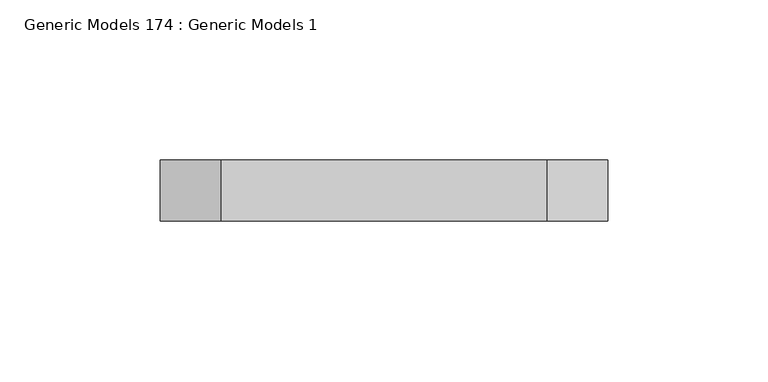
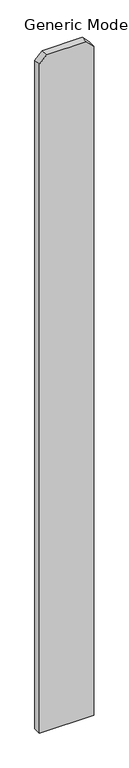
"""IFC4 building model written with IfcOpenShell, lengths in millimetres: proxy geometry, Generic Models 174 : Generic Models 1."""

import ifcopenshell
import ifcopenshell.guid

model = None  # the IFC model being written
_history = None  # IfcOwnerHistory: only IFC2X3 demands one
_inside = {}  # id of a spatial element -> (the spatial element, [elements in it])
_under = {}  # id of a project, library or spatial element -> (it, [spatial elements below it])
_declared = {}  # id of a project -> (the project, [libraries it declares])
_typed = {}  # id of a type object -> (the type object, [elements of that type])
_made_of = {}  # id of a material, layer set ... -> (it, [elements and type objects made of it])


def new_model(schema):
    """Start an empty IFC model of exactly this schema.

    Asked for "IFC4X3", IfcOpenShell would pick the latest addendum, in which some entities
    have other attributes; the version numbers below select the first issue.
    IFC2X3 requires an IfcOwnerHistory on every rooted entity: one is made here for all.
    """
    global model, _history
    if schema == "IFC4X3":
        model = ifcopenshell.file(schema_version=(4, 3, 0, 0))
    else:
        model = ifcopenshell.file(schema=schema)
    _inside.clear()
    _under.clear()
    _declared.clear()
    _typed.clear()
    _made_of.clear()
    _history = None
    if model.schema == "IFC2X3":
        org = make("IfcOrganization", Name="unknown")
        user = make(
            "IfcPersonAndOrganization",
            ThePerson=make("IfcPerson", FamilyName="unknown"),
            TheOrganization=org,
        )
        app = make(
            "IfcApplication",
            ApplicationDeveloper=org,
            Version="unknown",
            ApplicationFullName="unknown",
            ApplicationIdentifier="unknown",
        )
        _history = make(
            "IfcOwnerHistory",
            OwningUser=user,
            OwningApplication=app,
            ChangeAction="ADDED",
            CreationDate=0,
        )
    return model


def make(cls, **values):
    """One entity of the class cls with the attributes given. An attribute that is None is left unset."""
    return model.create_entity(
        cls, **{name: value for name, value in values.items() if value is not None}
    )


def rooted(cls, **values):
    """An entity with a GlobalId (a new one), such as an element, a storey or a relation."""
    return make(cls, GlobalId=ifcopenshell.guid.new(), OwnerHistory=_history, **values)


def si_unit(unit_type, name, prefix=None):
    """IfcSIUnit, for example si_unit("LENGTHUNIT", "METRE", prefix="MILLI")."""
    return make("IfcSIUnit", UnitType=unit_type, Prefix=prefix, Name=name)


def assignment(units):
    """IfcUnitAssignment: the units of a project."""
    return None if units is None else make("IfcUnitAssignment", Units=units)


def point(xyz):
    """IfcCartesianPoint."""
    return None if xyz is None else make("IfcCartesianPoint", Coordinates=xyz)


def direction(xyz):
    """IfcDirection."""
    return None if xyz is None else make("IfcDirection", DirectionRatios=xyz)


def frame(location, z_axis=None, x_axis=None):
    """IfcAxis2Placement3D, a coordinate frame: its origin and axes. An axis left out is left unset."""
    return make(
        "IfcAxis2Placement3D",
        Location=point(location),
        Axis=direction(z_axis),
        RefDirection=direction(x_axis),
    )


def origin():
    """The frame at (0, 0, 0) with its axes left unset."""
    return frame((0.0, 0.0, 0.0))


def place(relative_to, where):
    """IfcLocalPlacement: puts the frame where relative to a parent placement (None: the world)."""
    return make(
        "IfcLocalPlacement", PlacementRelTo=relative_to, RelativePlacement=where
    )


def context(
    kind, dimensions, precision=None, world=None, true_north=None, identifier=None
):
    """IfcGeometricRepresentationContext, for example the 3D "Model" context."""
    return make(
        "IfcGeometricRepresentationContext",
        ContextIdentifier=identifier,
        ContextType=kind,
        CoordinateSpaceDimension=dimensions,
        Precision=precision,
        WorldCoordinateSystem=world,
        TrueNorth=true_north,
    )


def project(units=None, contexts=None):
    """IfcProject with its units and contexts."""
    return rooted(
        "IfcProject",
        Name="project",
        RepresentationContexts=contexts,
        UnitsInContext=assignment(units),
    )


def spatial(cls, under=None, at=None, **own):
    """A site, building, storey or space (cls), placed at a placement, below another one or the project."""
    s = rooted(cls, ObjectPlacement=at, **own)
    if under is not None:
        _under.setdefault(under.id(), (under, []))[1].append(s)
    return s


def polyline(points):
    """IfcPolyline through the points."""
    return make("IfcPolyline", Points=[point(p) for p in points])


def outline(outer, holes=None, kind="AREA"):
    """IfcArbitraryClosedProfileDef: a profile drawn as a closed curve; with holes, ...WithVoids."""
    if holes is None:
        return make("IfcArbitraryClosedProfileDef", ProfileType=kind, OuterCurve=outer)
    return make(
        "IfcArbitraryProfileDefWithVoids",
        ProfileType=kind,
        OuterCurve=outer,
        InnerCurves=holes,
    )


def extrude(swept, where, along, depth):
    """IfcExtrudedAreaSolid: the profile swept, set in the frame where, extruded along a direction by depth."""
    return make(
        "IfcExtrudedAreaSolid",
        SweptArea=swept,
        Position=where,
        ExtrudedDirection=direction(along),
        Depth=depth,
    )


def shape(context_of_items, identifier, shape_type, items):
    """IfcShapeRepresentation: the items that make up one representation, for example the "Body"."""
    return make(
        "IfcShapeRepresentation",
        ContextOfItems=context_of_items,
        RepresentationIdentifier=identifier,
        RepresentationType=shape_type,
        Items=items,
    )


def source(mapping_origin, context_of_items, identifier, shape_type, items):
    """IfcRepresentationMap: a shape defined once, which mapped items show again and again."""
    return make(
        "IfcRepresentationMap",
        MappingOrigin=mapping_origin,
        MappedRepresentation=shape(context_of_items, identifier, shape_type, items),
    )


def transform(
    local_origin,
    x_axis=None,
    y_axis=None,
    z_axis=None,
    scale=None,
    scale2=None,
    scale3=None,
    uniform=True,
):
    """IfcCartesianTransformationOperator3D, or its non-uniform kind. x_axis, y_axis, z_axis: its Axis1, 2, 3."""
    if uniform:
        return make(
            "IfcCartesianTransformationOperator3D",
            Axis1=direction(x_axis),
            Axis2=direction(y_axis),
            LocalOrigin=point(local_origin),
            Scale=scale,
            Axis3=direction(z_axis),
        )
    return make(
        "IfcCartesianTransformationOperator3DnonUniform",
        Axis1=direction(x_axis),
        Axis2=direction(y_axis),
        LocalOrigin=point(local_origin),
        Scale=scale,
        Axis3=direction(z_axis),
        Scale2=scale2,
        Scale3=scale3,
    )


def mapped(mapping_source, mapping_target):
    """IfcMappedItem: shows the shape of a source again, moved by a transform."""
    return make(
        "IfcMappedItem", MappingSource=mapping_source, MappingTarget=mapping_target
    )


def made_of(thing, what):
    """Note that an element or type object is made of a material, layer set ...; save() writes the relation."""
    if what is not None:
        _made_of.setdefault(what.id(), (what, []))[1].append(thing)
    return thing


def element(
    cls,
    number,
    at=None,
    inside=None,
    cuts=None,
    type_object=None,
    material=None,
    context=None,
    identifier="Body",
    shape_type=None,
    held_by="IfcProductDefinitionShape",
    body=None,
    shapes=None,
    **own,
):
    """One element of the class cls, such as IfcWall. Its Tag is "e" and its number.

    at: its placement. inside: the storey or other place that contains it. cuts: it is an
    opening in that element (IfcRelVoidsElement). A single representation is given by context,
    identifier, shape_type and body (its items); several are given by shapes. held_by: the class
    of the entity that holds the representations. save() writes the other relations.
    """
    e = rooted(cls, Tag="e%d" % number, ObjectPlacement=at, **own)
    if body is not None:
        shapes = [shape(context, identifier, shape_type, body)]
    if shapes is not None:
        e.Representation = make(held_by, Representations=shapes)
    if inside is not None:
        _inside.setdefault(inside.id(), (inside, []))[1].append(e)
    if cuts is not None:
        rooted(
            "IfcRelVoidsElement", RelatingBuildingElement=cuts, RelatedOpeningElement=e
        )
    if type_object is not None:
        _typed.setdefault(type_object.id(), (type_object, []))[1].append(e)
    return made_of(e, material)


def aggregate(whole, parts):
    """IfcRelAggregates: a whole, such as a stair, and the parts it consists of."""
    return rooted("IfcRelAggregates", RelatingObject=whole, RelatedObjects=parts)


def save(model, path):
    """Write the relations noted so far, then the file.

    IfcRelAggregates (storeys below a building ...), IfcRelContainedInSpatialStructure (elements
    in a storey), IfcRelDefinesByType, IfcRelAssociatesMaterial and IfcRelDeclares: one each for
    every whole, place, type object, material and project.
    """
    for whole, parts in _under.values():
        aggregate(whole, parts)
    for where, things in _inside.values():
        rooted(
            "IfcRelContainedInSpatialStructure",
            RelatedElements=things,
            RelatingStructure=where,
        )
    for kind, things in _typed.values():
        rooted("IfcRelDefinesByType", RelatedObjects=things, RelatingType=kind)
    for what, things in _made_of.values():
        rooted("IfcRelAssociatesMaterial", RelatedObjects=things, RelatingMaterial=what)
    for by, libraries in _declared.values():
        rooted("IfcRelDeclares", RelatingContext=by, RelatedDefinitions=libraries)
    model.write(path)


def generic_models_174_generic_models_1_c9b0eb3d(model_context):
    return source(origin(), model_context, "Body", "SweptSolid", [
        extrude(outline(polyline([(76.2, 56513.4125), (1885.95, 56513.4125), (1905.0, 56494.3625), (1905.0, 56392.7625), (1885.95, 56373.7125), (76.2, 56373.7125), (76.2, 56513.4125)])), frame((0.0, 547.6875, 0.0), z_axis=(0.0, 1.0, 0.0), x_axis=(0.0, 0.0, 1.0)), (0.0, 0.0, 1.0), 19.05),
    ])


if __name__ == "__main__":
    model = new_model("IFC4")
    model_context = context("Model", 3, world=origin())
    ifc_project = project(units=[si_unit("LENGTHUNIT", "METRE", prefix="MILLI")], contexts=[model_context])
    site = spatial("IfcSite", under=ifc_project)
    building = spatial("IfcBuilding", under=site)
    placement = place(None, origin())
    generic_models_174_generic_models_1_shape = generic_models_174_generic_models_1_c9b0eb3d(model_context)
    element("IfcBuildingElementProxy", 1, Name="Generic Models 174 : Generic Models 1", ObjectType="Generic Models 174 : Generic Models 1", at=placement, inside=building, context=model_context, shape_type="MappedRepresentation", body=[
        mapped(generic_models_174_generic_models_1_shape, transform((0.0, 0.0, 0.0), x_axis=(1.0, 0.0, 0.0), y_axis=(0.0, 1.0, 0.0), z_axis=(0.0, 0.0, 1.0))),
    ])
    save(model, "model.ifc")

# Revit data of these elements
# Element 1 (IfcBuildingElementProxy, "Generic Models 174 : Generic Models 1")
#   Materials on its faces: "VERTICAL 1X6 CEDAR PLANKS W/ CLEAR WOOD SEALER"
# Materials
#   "VERTICAL 1X6 CEDAR PLANKS W/ CLEAR WOOD SEALER": class "Wood", colour RGB 234 198 147, transparency 0, Description = "Pinus Echinata", Cost = 0
